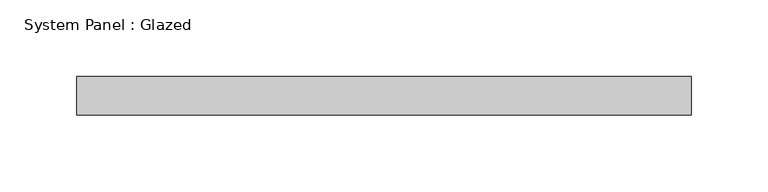
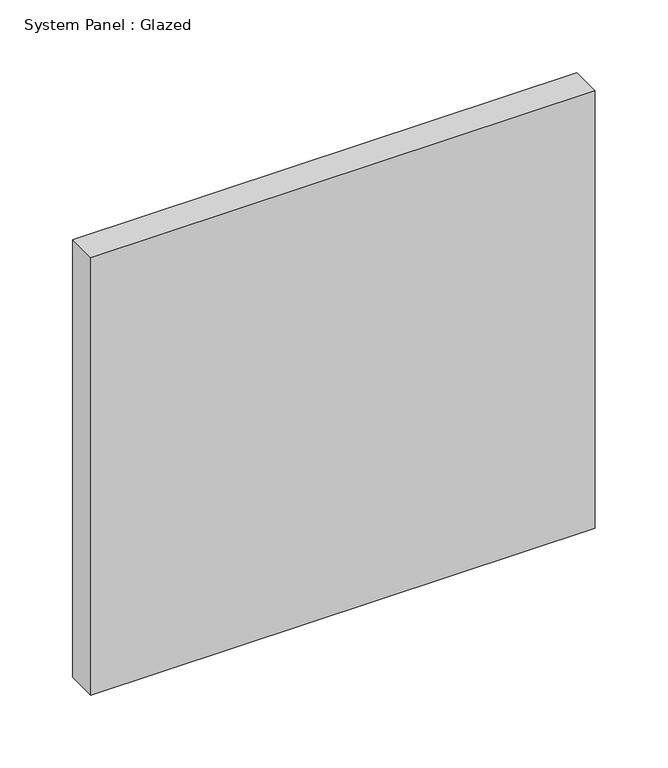
"""IFC4 building model written with IfcOpenShell, lengths in millimetres: plate geometry, System Panel : Glazed."""

from ifc_helpers import new_model, si_unit, origin, origin_with_axes, place, context, project, spatial, polyline, outline, extrude, source, transform, mapped, element, save


def system_panel_glazed_fa4770cb(model_context):
    return source(origin(), model_context, "Body", "SweptSolid", [
        extrude(outline(polyline([(200.0, 24.5), (-200.0, 24.5), (-200.0, 49.5), (200.0, 49.5), (200.0, 24.5)])), origin_with_axes(), (0.0, 0.0, 1.0), 366.6666667),
    ])


if __name__ == "__main__":
    model = new_model("IFC4")
    model_context = context("Model", 3, world=origin())
    ifc_project = project(units=[si_unit("LENGTHUNIT", "METRE", prefix="MILLI")], contexts=[model_context])
    site = spatial("IfcSite", under=ifc_project)
    building = spatial("IfcBuilding", under=site)
    placement = place(None, origin())
    system_panel_glazed_shape = system_panel_glazed_fa4770cb(model_context)
    element("IfcPlate", 1, ObjectType="System Panel : Glazed", at=placement, inside=building, context=model_context, shape_type="MappedRepresentation", body=[
        mapped(system_panel_glazed_shape, transform((0.0, 0.0, 0.0), x_axis=(1.0, 0.0, 0.0), y_axis=(0.0, 1.0, 0.0), z_axis=(0.0, 0.0, 1.0))),
    ])
    save(model, "model.ifc")

# Revit data of these elements
# Element 1 (IfcPlate, "System Panel : Glazed")
#   Materials on its faces: "Glass"
# Materials
#   "Glass": class "Glass", colour RGB 218 227 224, transparency 0.85, Description = "Soda Lime Glass", Cost = 0
